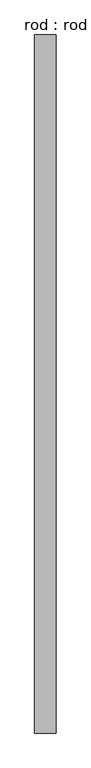
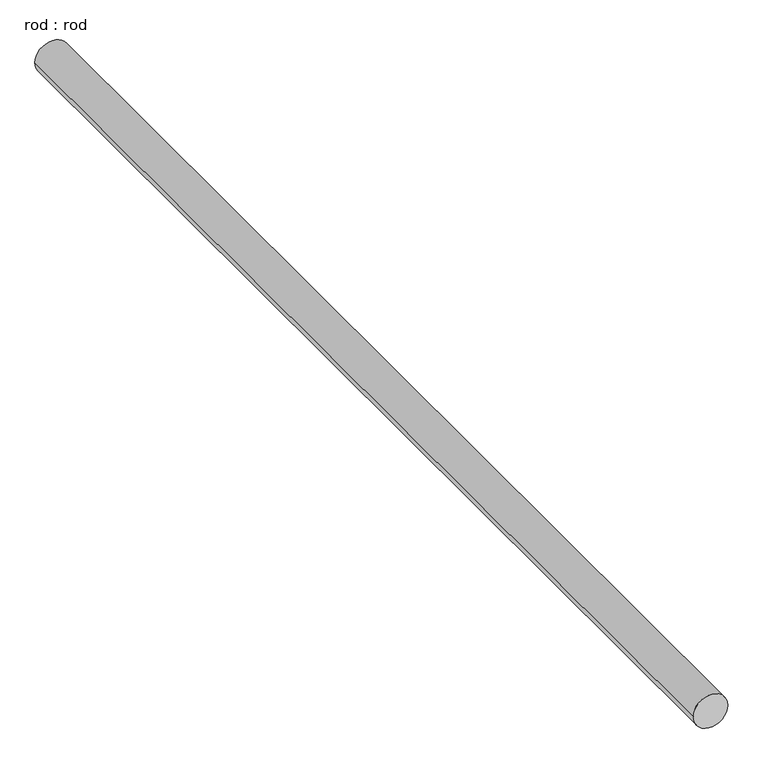
"""IFC4 building model written with IfcOpenShell, lengths in millimetres: proxy geometry, rod : rod."""

from ifc_helpers import new_model, si_unit, point, frame, frame_2d, origin, place, context, project, spatial, circle_curve, trimmed, segment, composite_curve, outline, extrude, source, transform, mapped, element, save


def rod_rod_359df746(model_context):
    return source(origin(), model_context, "Body", "SweptSolid", [
        extrude(outline(composite_curve([segment(trimmed(circle_curve(frame_2d((0.0108462, 0.0)), 200.0), [point((0.0108462, 200.0))], [point((0.0108462, -200.0))], False, "CARTESIAN"), True, "CONTINUOUS"), segment(trimmed(circle_curve(frame_2d((0.0108462, 0.0)), 200.0), [point((0.0108462, -200.0))], [point((0.0108462, 200.0))], False, "CARTESIAN"), True, "CONTINUOUS")], self_intersect=False)), frame((0.0, -2490.5247754, 0.0), z_axis=(0.0, 1.0, 0.0), x_axis=(0.0, 0.0, 1.0)), (0.0, 0.0, 1.0), 13166.5067815),
    ])


if __name__ == "__main__":
    model = new_model("IFC4")
    model_context = context("Model", 3, world=origin())
    ifc_project = project(units=[si_unit("LENGTHUNIT", "METRE", prefix="MILLI")], contexts=[model_context])
    site = spatial("IfcSite", under=ifc_project)
    building = spatial("IfcBuilding", under=site)
    placement = place(None, origin())
    rod_rod_shape = rod_rod_359df746(model_context)
    element("IfcBuildingElementProxy", 1, Name="rod : rod", ObjectType="rod : rod", at=placement, inside=building, context=model_context, shape_type="MappedRepresentation", body=[
        mapped(rod_rod_shape, transform((0.0, 0.0, 0.0), x_axis=(1.0, 0.0, 0.0), y_axis=(0.0, 1.0, 0.0), z_axis=(0.0, 0.0, 1.0))),
    ])
    save(model, "model.ifc")

# Revit data of these elements
# Type "rod : rod"
#   Default Elevation = 0
